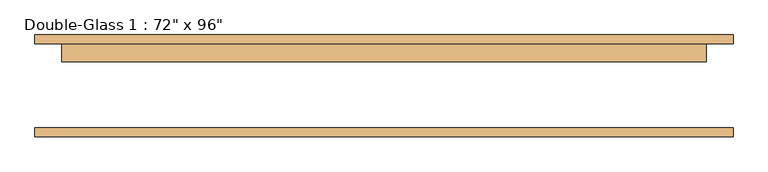
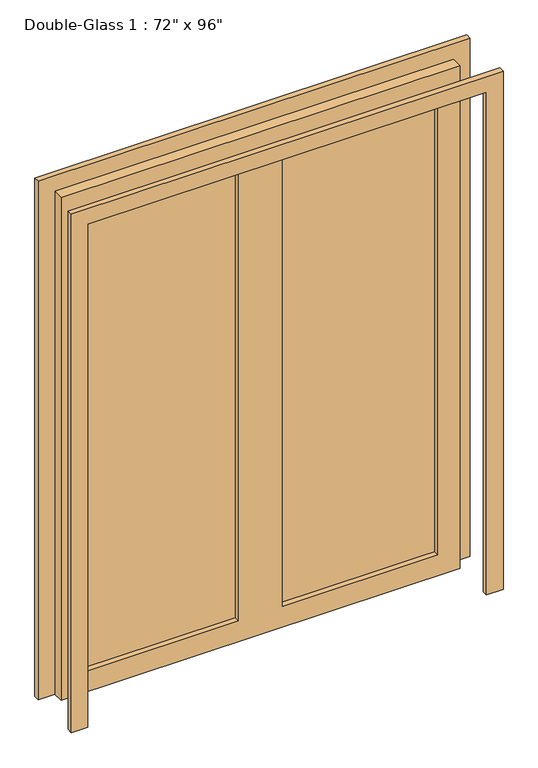
"""IFC4 building model written with IfcOpenShell, lengths in millimetres: door geometry."""

from ifc_helpers import new_model, si_unit, frame, origin, place, context, project, spatial, polyline, outline, extrude, source, transform, mapped, element, save


def door_b24398f5(model_context):
    return source(origin(), model_context, "Body", "SweptSolid", [
        extrude(outline(polyline([(0.0, 990.6), (2514.6, 990.6), (2514.6, -990.6), (0.0, -990.6), (0.0, -914.4), (2438.4, -914.4), (2438.4, 914.4), (0.0, 914.4), (0.0, 990.6)])), frame((0.0, -142.08125, 0.0), z_axis=(0.0, 1.0, 0.0), x_axis=(0.0, 0.0, 1.0)), (0.0, 0.0, 1.0), 25.4),
        extrude(outline(polyline([(2438.4, 914.4), (0.0, 914.4), (0.0, 990.6), (2514.6, 990.6), (2514.6, -990.6), (0.0, -990.6), (0.0, -914.4), (2438.4, -914.4), (2438.4, 914.4)])), frame((0.0, 121.44375, 0.0), z_axis=(0.0, 1.0, 0.0), x_axis=(0.0, 0.0, 1.0)), (0.0, 0.0, 1.0), 25.4),
        extrude(outline(polyline([(812.8, 96.04375), (101.6, 96.04375), (101.6, 103.1875), (812.8, 103.1875), (812.8, 96.04375)])), frame((0.0, 0.0, 101.6), z_axis=(0.0, 0.0, 1.0), x_axis=(1.0, 0.0, 0.0)), (0.0, 0.0, 1.0), 2235.2),
        extrude(outline(polyline([(-101.6, 96.04375), (-812.8, 96.04375), (-812.8, 103.1875), (-101.6, 103.1875), (-101.6, 96.04375)])), frame((0.0, 0.0, 101.6), z_axis=(0.0, 0.0, 1.0), x_axis=(1.0, 0.0, 0.0)), (0.0, 0.0, 1.0), 2235.2),
        extrude(outline(polyline([(2438.4, 914.4), (2438.4, -914.4), (0.0, -914.4), (0.0, 914.4), (2438.4, 914.4)]), holes=[polyline([(2336.8, -101.6), (101.6, -101.6), (101.6, -812.8), (2336.8, -812.8), (2336.8, -101.6)]), polyline([(2336.8, 812.8), (101.6, 812.8), (101.6, 101.6), (2336.8, 101.6), (2336.8, 812.8)])]), frame((0.0, 70.64375, 0.0), z_axis=(0.0, 1.0, 0.0), x_axis=(0.0, 0.0, 1.0)), (0.0, 0.0, 1.0), 50.8),
    ])


if __name__ == "__main__":
    model = new_model("IFC4")
    model_context = context("Model", 3, world=origin())
    ifc_project = project(units=[si_unit("LENGTHUNIT", "METRE", prefix="MILLI")], contexts=[model_context])
    site = spatial("IfcSite", under=ifc_project)
    building = spatial("IfcBuilding", under=site)
    placement = place(None, origin())
    door_shape = door_b24398f5(model_context)
    element("IfcDoor", 1, ObjectType="Double-Glass 1 : 72\" x 96\"", at=placement, inside=building, context=model_context, shape_type="MappedRepresentation", body=[
        mapped(door_shape, transform((0.0, 0.0, 0.0), x_axis=(1.0, 0.0, 0.0), y_axis=(0.0, 1.0, 0.0), z_axis=(0.0, 0.0, 1.0))),
    ])
    save(model, "model.ifc")

# Revit data of these elements
# Type "Double-Glass 1 : 72\" x 96\""
#   Type Mark = "30"
#   Construction Type Id = "MDOOR"
#   Assembly Code = "C1020"
#   Analytic Construction = "Metal"
#   Thickness = 0' - 2"
#   Thermal Resistance (R) = 0.270118 (m²·K)/W
#   Heat Transfer Coefficient (U) = 3.70223 W/(m²·K)
#   Height = 8' - 0"
#   Rail Width - Base = 0' - 4"
#   Rail Width - Top = 0' - 4"
#   Stile Width - Hinge = 0' - 4"
#   Stile Width - Latch = 0' - 4"
#   Trim Projection = 0' - 1"
#   Trim Width = 0' - 3"
#   Width = 6' - 0"
#   Door Material = Aluminum
#   Frame Material = Aluminum
#   Visual Light Transmittance = 0
#   Solar Heat Gain Coefficient = 0
#   Function = (empty or 0)
#   Wall Closure = (empty or 0)
# Element 1 (IfcDoor, "Double-Glass 1 : 72\" x 96\"")
#   Materials on its faces: "Aluminum", "Glass"
# Materials
#   "Aluminum": class "Metal", colour RGB 247 247 247, transparency 0, Description = "Aluminum 6061", Cost = 0
#   "Glass": class "Glass", colour RGB 0 128 192, transparency 0.75, Description = "Soda Lime Glass", Cost = 0
